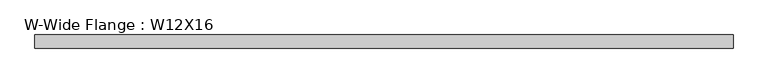
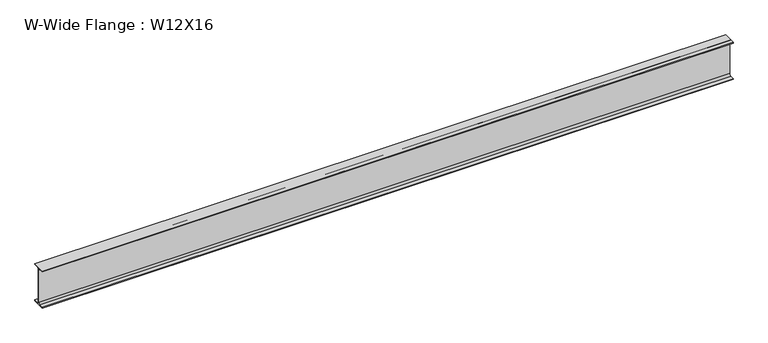
"""IFC4 building model written with IfcOpenShell, lengths in millimetres: beam geometry, W-Wide Flange : W12X16."""

from ifc_helpers import new_model, si_unit, point, frame, frame_2d, origin, place, context, project, spatial, polyline, circle_curve, trimmed, segment, composite_curve, outline, extrude, source, transform, mapped, element, save


def w_wide_flange_w12x16_53d9ec52(model_context):
    return source(origin(), model_context, "Body", "SweptSolid", [
        extrude(outline(composite_curve([segment(polyline([(50.673, -145.669), (50.673, -152.4), (-50.673, -152.4), (-50.673, -145.669), (-16.7005, -145.669)]), True, "CONTINUOUS"), segment(trimmed(circle_curve(frame_2d((-16.7005, -131.7625)), 13.9065), [point((-16.7005, -145.669))], [point((-2.794, -131.7625))], True, "CARTESIAN"), True, "CONTINUOUS"), segment(polyline([(-2.794, -131.7625), (-2.794, 131.7625)]), True, "CONTINUOUS"), segment(trimmed(circle_curve(frame_2d((-16.7005, 131.7625)), 13.9065), [point((-2.794, 131.7625))], [point((-16.7005, 145.669))], True, "CARTESIAN"), True, "CONTINUOUS"), segment(polyline([(-16.7005, 145.669), (-50.673, 145.669), (-50.673, 152.4), (50.673, 152.4), (50.673, 145.669), (16.7005, 145.669)]), True, "CONTINUOUS"), segment(trimmed(circle_curve(frame_2d((16.7005, 131.7625)), 13.9065), [point((16.7005, 145.669))], [point((2.794, 131.7625))], True, "CARTESIAN"), True, "CONTINUOUS"), segment(polyline([(2.794, 131.7625), (2.794, -131.7625)]), True, "CONTINUOUS"), segment(trimmed(circle_curve(frame_2d((16.7005, -131.7625)), 13.9065), [point((2.794, -131.7625))], [point((16.7005, -145.669))], True, "CARTESIAN"), True, "CONTINUOUS"), segment(polyline([(16.7005, -145.669), (50.673, -145.669)]), True, "CONTINUOUS")], self_intersect=False)), frame((-2692.527, 0.0, 0.0), z_axis=(1.0, 0.0, 0.0), x_axis=(0.0, 1.0, 0.0)), (0.0, 0.0, 1.0), 5385.054),
    ])


if __name__ == "__main__":
    model = new_model("IFC4")
    model_context = context("Model", 3, world=origin())
    ifc_project = project(units=[si_unit("LENGTHUNIT", "METRE", prefix="MILLI")], contexts=[model_context])
    site = spatial("IfcSite", under=ifc_project)
    building = spatial("IfcBuilding", under=site)
    placement = place(None, origin())
    w_wide_flange_w12x16_shape = w_wide_flange_w12x16_53d9ec52(model_context)
    element("IfcBeam", 1, ObjectType="W-Wide Flange : W12X16", at=placement, inside=building, context=model_context, shape_type="MappedRepresentation", body=[
        mapped(w_wide_flange_w12x16_shape, transform((0.0, 0.0, 0.0), x_axis=(1.0, 0.0, 0.0), y_axis=(0.0, 1.0, 0.0), z_axis=(0.0, 0.0, 1.0))),
    ])
    save(model, "model.ifc")

# Revit data of these elements
# Type "W-Wide Flange : W12X16"
#   Assembly Code = "B10"
#   W = 16
#   Length [instance default] = 5' - 0"
#   bf = 0' - 3.99"
#   d = 1' - 0"
#   k = 0' - 0 13/16"
#   k2 = 0' - 0.5475"
#   tf = 0' - 0.265"
#   tw = 0' - 0.22"
#   A = 0.0327083 SF
#   Structural Material [instance default] = Steel ASTM A992
# Element 1 (IfcBeam, "W-Wide Flange : W12X16")
#   Structural Material = Steel ASTM A36
#   Materials on its faces: "Steel ASTM A36"
# Materials
#   "Steel ASTM A992": class "Metal", colour RGB 199 199 199, transparency 0, Description = "Structural steel 50ksi", Cost = 0
#   "Steel ASTM A36": class "Metal", colour RGB 199 199 199, transparency 0, Description = "Structural steel, ASTM A36 Grade B, mill finish", Cost = 0
